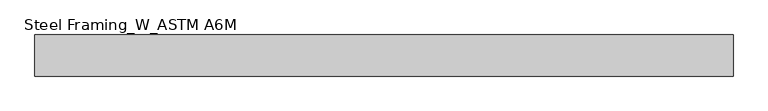
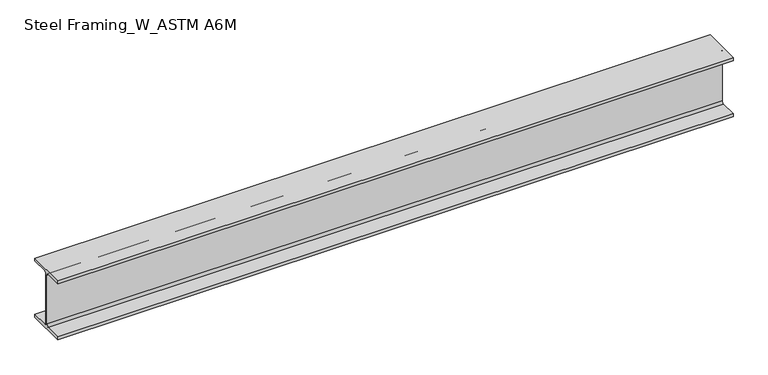
"""IFC4 building model written with IfcOpenShell, lengths in millimetres: beam geometry, Steel Framing_W_ASTM A6M : H_SB_AR_S02_W200x31.3_B6."""

from ifc_helpers import new_model, si_unit, point, frame, frame_2d, origin, place, context, project, spatial, polyline, circle_curve, trimmed, segment, composite_curve, outline, extrude, source, transform, mapped, element, save


def steel_framing_w_astm_a6m_8355ed91(model_context):
    return source(origin(), model_context, "Body", "SweptSolid", [
        extrude(outline(composite_curve([segment(polyline([(67.0, -94.8), (67.0, -105.0), (-67.0, -105.0), (-67.0, -94.8), (-10.775, -94.8)]), True, "CONTINUOUS"), segment(trimmed(circle_curve(frame_2d((-10.775, -87.2)), 7.6), [point((-10.775, -94.8))], [point((-3.175, -87.2))], True, "CARTESIAN"), True, "CONTINUOUS"), segment(polyline([(-3.175, -87.2), (-3.175, 87.2)]), True, "CONTINUOUS"), segment(trimmed(circle_curve(frame_2d((-10.775, 87.2)), 7.6), [point((-3.175, 87.2))], [point((-10.775, 94.8))], True, "CARTESIAN"), True, "CONTINUOUS"), segment(polyline([(-10.775, 94.8), (-67.0, 94.8), (-67.0, 105.0), (67.0, 105.0), (67.0, 94.8), (10.775, 94.8)]), True, "CONTINUOUS"), segment(trimmed(circle_curve(frame_2d((10.775, 87.2)), 7.6), [point((10.775, 94.8))], [point((3.175, 87.2))], True, "CARTESIAN"), True, "CONTINUOUS"), segment(polyline([(3.175, 87.2), (3.175, -87.2)]), True, "CONTINUOUS"), segment(trimmed(circle_curve(frame_2d((10.775, -87.2)), 7.6), [point((3.175, -87.2))], [point((10.775, -94.8))], True, "CARTESIAN"), True, "CONTINUOUS"), segment(polyline([(10.775, -94.8), (67.0, -94.8)]), True, "CONTINUOUS")], self_intersect=False)), frame((-1136.3, 0.0, 0.0), z_axis=(1.0, 0.0, 0.0), x_axis=(0.0, 1.0, 0.0)), (0.0, 0.0, 1.0), 2272.6),
    ])


if __name__ == "__main__":
    model = new_model("IFC4")
    model_context = context("Model", 3, world=origin())
    ifc_project = project(units=[si_unit("LENGTHUNIT", "METRE", prefix="MILLI")], contexts=[model_context])
    site = spatial("IfcSite", under=ifc_project)
    building = spatial("IfcBuilding", under=site)
    placement = place(None, origin())
    steel_framing_w_astm_a6m_shape = steel_framing_w_astm_a6m_8355ed91(model_context)
    element("IfcBeam", 1, ObjectType="Steel Framing_W_ASTM A6M : H_SB_AR_S02_W200x31.3_B6", at=placement, inside=building, context=model_context, shape_type="MappedRepresentation", body=[
        mapped(steel_framing_w_astm_a6m_shape, transform((0.0, 0.0, 0.0), x_axis=(1.0, 0.0, 0.0), y_axis=(0.0, 1.0, 0.0), z_axis=(0.0, 0.0, 1.0))),
    ])
    save(model, "model.ifc")

# Revit data of these elements
# Type "Steel Framing_W_ASTM A6M : H_SB_AR_S02_W200x31.3_B6"
#   Type Mark = "B6"
#   Section Name Key = "W8x21"
#   Width = 13.4 cm
#   Web Thickness = 0.635 cm
#   Web Fillet = 0.76 cm
#   Warping Constant = 40800.0 cm⁶
#   Torsional Moment of Inertia = 11.70 cm⁴
#   Section Area = 39.7 cm²
#   Plastic Modulus weak axis = 93.2 cm³
#   Plastic Modulus strong axis = 334.0 cm³
#   Perimeter = 0.93 m²/m
#   Nominal Weight = 31.30 kgf/m
#   Moment of Inertia weak axis = 407.00 cm⁴
#   Moment of Inertia strong axis = 3130.00 cm⁴
#   Height = 21.0 cm
#   Flange Thickness = 1.02 cm
#   Elastic Modulus weak axis = 60.8 cm³
#   Elastic Modulus strong axis = 298.0 cm³
#   Centroid Vertical = 10.5 cm
#   Centroid Horizontal = 6.7 cm
#   Length [instance default] = 1500 mm
#   Structural Material [instance default] = Steel, 45-345
#   Bolt Spacing = 0
#   Assembly Code = ""
# Element 1 (IfcBeam, "Steel Framing_W_ASTM A6M : H_SB_AR_S02_W200x31.3_B6")
#   Materials on its faces: "Steel, 45-345"
# Materials
#   "Steel, 45-345": class "Metal", colour RGB 189 187 185, transparency 0, Description = "Steel 345 MPa", Cost = 0
